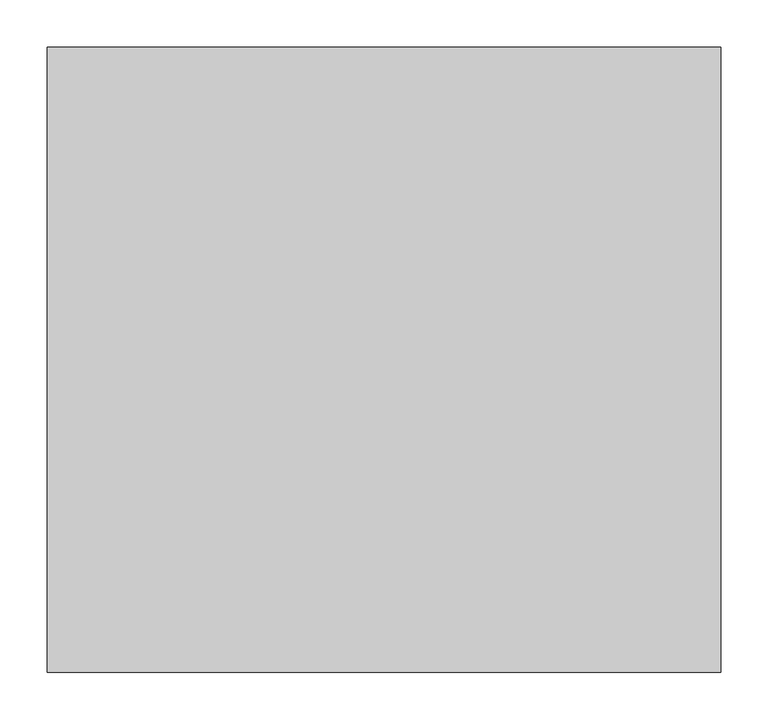
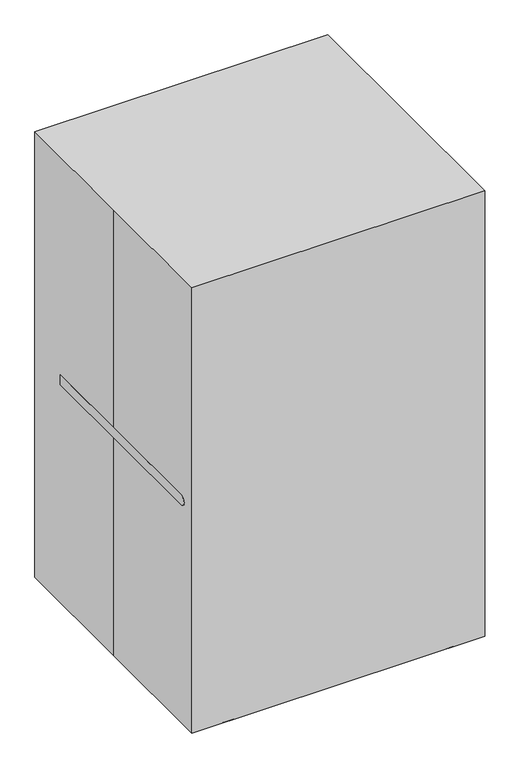
"""IFC4 building model written with IfcOpenShell, lengths in millimetres: proxy geometry, F0270 - Chair, Rocking, High Back : F0270 - Chair, Rocking, High Back."""

import ifcopenshell
import ifcopenshell.guid

model = None  # the IFC model being written
_history = None  # IfcOwnerHistory: only IFC2X3 demands one
_inside = {}  # id of a spatial element -> (the spatial element, [elements in it])
_under = {}  # id of a project, library or spatial element -> (it, [spatial elements below it])
_declared = {}  # id of a project -> (the project, [libraries it declares])
_typed = {}  # id of a type object -> (the type object, [elements of that type])
_made_of = {}  # id of a material, layer set ... -> (it, [elements and type objects made of it])


def new_model(schema):
    """Start an empty IFC model of exactly this schema.

    Asked for "IFC4X3", IfcOpenShell would pick the latest addendum, in which some entities
    have other attributes; the version numbers below select the first issue.
    IFC2X3 requires an IfcOwnerHistory on every rooted entity: one is made here for all.
    """
    global model, _history
    if schema == "IFC4X3":
        model = ifcopenshell.file(schema_version=(4, 3, 0, 0))
    else:
        model = ifcopenshell.file(schema=schema)
    _inside.clear()
    _under.clear()
    _declared.clear()
    _typed.clear()
    _made_of.clear()
    _history = None
    if model.schema == "IFC2X3":
        org = make("IfcOrganization", Name="unknown")
        user = make(
            "IfcPersonAndOrganization",
            ThePerson=make("IfcPerson", FamilyName="unknown"),
            TheOrganization=org,
        )
        app = make(
            "IfcApplication",
            ApplicationDeveloper=org,
            Version="unknown",
            ApplicationFullName="unknown",
            ApplicationIdentifier="unknown",
        )
        _history = make(
            "IfcOwnerHistory",
            OwningUser=user,
            OwningApplication=app,
            ChangeAction="ADDED",
            CreationDate=0,
        )
    return model


def make(cls, **values):
    """One entity of the class cls with the attributes given. An attribute that is None is left unset."""
    return model.create_entity(
        cls, **{name: value for name, value in values.items() if value is not None}
    )


def rooted(cls, **values):
    """An entity with a GlobalId (a new one), such as an element, a storey or a relation."""
    return make(cls, GlobalId=ifcopenshell.guid.new(), OwnerHistory=_history, **values)


def si_unit(unit_type, name, prefix=None):
    """IfcSIUnit, for example si_unit("LENGTHUNIT", "METRE", prefix="MILLI")."""
    return make("IfcSIUnit", UnitType=unit_type, Prefix=prefix, Name=name)


def assignment(units):
    """IfcUnitAssignment: the units of a project."""
    return None if units is None else make("IfcUnitAssignment", Units=units)


def point(xyz):
    """IfcCartesianPoint."""
    return None if xyz is None else make("IfcCartesianPoint", Coordinates=xyz)


def direction(xyz):
    """IfcDirection."""
    return None if xyz is None else make("IfcDirection", DirectionRatios=xyz)


def frame(location, z_axis=None, x_axis=None):
    """IfcAxis2Placement3D, a coordinate frame: its origin and axes. An axis left out is left unset."""
    return make(
        "IfcAxis2Placement3D",
        Location=point(location),
        Axis=direction(z_axis),
        RefDirection=direction(x_axis),
    )


def frame_2d(location, x_axis=None):
    """IfcAxis2Placement2D, a coordinate frame in the plane: its origin and x axis."""
    return make(
        "IfcAxis2Placement2D", Location=point(location), RefDirection=direction(x_axis)
    )


def origin():
    """The frame at (0, 0, 0) with its axes left unset."""
    return frame((0.0, 0.0, 0.0))


def origin_with_axes():
    """The frame at (0, 0, 0) with the z axis (0, 0, 1) and the x axis (1, 0, 0) written out."""
    return frame((0.0, 0.0, 0.0), z_axis=(0.0, 0.0, 1.0), x_axis=(1.0, 0.0, 0.0))


def place(relative_to, where):
    """IfcLocalPlacement: puts the frame where relative to a parent placement (None: the world)."""
    return make(
        "IfcLocalPlacement", PlacementRelTo=relative_to, RelativePlacement=where
    )


def context(
    kind, dimensions, precision=None, world=None, true_north=None, identifier=None
):
    """IfcGeometricRepresentationContext, for example the 3D "Model" context."""
    return make(
        "IfcGeometricRepresentationContext",
        ContextIdentifier=identifier,
        ContextType=kind,
        CoordinateSpaceDimension=dimensions,
        Precision=precision,
        WorldCoordinateSystem=world,
        TrueNorth=true_north,
    )


def project(units=None, contexts=None):
    """IfcProject with its units and contexts."""
    return rooted(
        "IfcProject",
        Name="project",
        RepresentationContexts=contexts,
        UnitsInContext=assignment(units),
    )


def spatial(cls, under=None, at=None, **own):
    """A site, building, storey or space (cls), placed at a placement, below another one or the project."""
    s = rooted(cls, ObjectPlacement=at, **own)
    if under is not None:
        _under.setdefault(under.id(), (under, []))[1].append(s)
    return s


def polyline(points):
    """IfcPolyline through the points."""
    return make("IfcPolyline", Points=[point(p) for p in points])


def circle_curve(where, radius):
    """IfcCircle in the frame where."""
    return make("IfcCircle", Position=where, Radius=radius)


def trimmed(basis, trim1, trim2, sense, master):
    """IfcTrimmedCurve: the piece of a basis curve between two trims."""
    return make(
        "IfcTrimmedCurve",
        BasisCurve=basis,
        Trim1=trim1,
        Trim2=trim2,
        SenseAgreement=sense,
        MasterRepresentation=master,
    )


def segment(curve, same_sense, transition):
    """IfcCompositeCurveSegment."""
    return make(
        "IfcCompositeCurveSegment",
        Transition=transition,
        SameSense=same_sense,
        ParentCurve=curve,
    )


def composite_curve(segments, self_intersect=None):
    """IfcCompositeCurve: segments joined end to end."""
    return make("IfcCompositeCurve", Segments=segments, SelfIntersect=self_intersect)


def outline(outer, holes=None, kind="AREA"):
    """IfcArbitraryClosedProfileDef: a profile drawn as a closed curve; with holes, ...WithVoids."""
    if holes is None:
        return make("IfcArbitraryClosedProfileDef", ProfileType=kind, OuterCurve=outer)
    return make(
        "IfcArbitraryProfileDefWithVoids",
        ProfileType=kind,
        OuterCurve=outer,
        InnerCurves=holes,
    )


def extrude(swept, where, along, depth):
    """IfcExtrudedAreaSolid: the profile swept, set in the frame where, extruded along a direction by depth."""
    return make(
        "IfcExtrudedAreaSolid",
        SweptArea=swept,
        Position=where,
        ExtrudedDirection=direction(along),
        Depth=depth,
    )


def shape(context_of_items, identifier, shape_type, items):
    """IfcShapeRepresentation: the items that make up one representation, for example the "Body"."""
    return make(
        "IfcShapeRepresentation",
        ContextOfItems=context_of_items,
        RepresentationIdentifier=identifier,
        RepresentationType=shape_type,
        Items=items,
    )


def source(mapping_origin, context_of_items, identifier, shape_type, items):
    """IfcRepresentationMap: a shape defined once, which mapped items show again and again."""
    return make(
        "IfcRepresentationMap",
        MappingOrigin=mapping_origin,
        MappedRepresentation=shape(context_of_items, identifier, shape_type, items),
    )


def transform(
    local_origin,
    x_axis=None,
    y_axis=None,
    z_axis=None,
    scale=None,
    scale2=None,
    scale3=None,
    uniform=True,
):
    """IfcCartesianTransformationOperator3D, or its non-uniform kind. x_axis, y_axis, z_axis: its Axis1, 2, 3."""
    if uniform:
        return make(
            "IfcCartesianTransformationOperator3D",
            Axis1=direction(x_axis),
            Axis2=direction(y_axis),
            LocalOrigin=point(local_origin),
            Scale=scale,
            Axis3=direction(z_axis),
        )
    return make(
        "IfcCartesianTransformationOperator3DnonUniform",
        Axis1=direction(x_axis),
        Axis2=direction(y_axis),
        LocalOrigin=point(local_origin),
        Scale=scale,
        Axis3=direction(z_axis),
        Scale2=scale2,
        Scale3=scale3,
    )


def mapped(mapping_source, mapping_target):
    """IfcMappedItem: shows the shape of a source again, moved by a transform."""
    return make(
        "IfcMappedItem", MappingSource=mapping_source, MappingTarget=mapping_target
    )


def made_of(thing, what):
    """Note that an element or type object is made of a material, layer set ...; save() writes the relation."""
    if what is not None:
        _made_of.setdefault(what.id(), (what, []))[1].append(thing)
    return thing


def element(
    cls,
    number,
    at=None,
    inside=None,
    cuts=None,
    type_object=None,
    material=None,
    context=None,
    identifier="Body",
    shape_type=None,
    held_by="IfcProductDefinitionShape",
    body=None,
    shapes=None,
    **own,
):
    """One element of the class cls, such as IfcWall. Its Tag is "e" and its number.

    at: its placement. inside: the storey or other place that contains it. cuts: it is an
    opening in that element (IfcRelVoidsElement). A single representation is given by context,
    identifier, shape_type and body (its items); several are given by shapes. held_by: the class
    of the entity that holds the representations. save() writes the other relations.
    """
    e = rooted(cls, Tag="e%d" % number, ObjectPlacement=at, **own)
    if body is not None:
        shapes = [shape(context, identifier, shape_type, body)]
    if shapes is not None:
        e.Representation = make(held_by, Representations=shapes)
    if inside is not None:
        _inside.setdefault(inside.id(), (inside, []))[1].append(e)
    if cuts is not None:
        rooted(
            "IfcRelVoidsElement", RelatingBuildingElement=cuts, RelatedOpeningElement=e
        )
    if type_object is not None:
        _typed.setdefault(type_object.id(), (type_object, []))[1].append(e)
    return made_of(e, material)


def aggregate(whole, parts):
    """IfcRelAggregates: a whole, such as a stair, and the parts it consists of."""
    return rooted("IfcRelAggregates", RelatingObject=whole, RelatedObjects=parts)


def save(model, path):
    """Write the relations noted so far, then the file.

    IfcRelAggregates (storeys below a building ...), IfcRelContainedInSpatialStructure (elements
    in a storey), IfcRelDefinesByType, IfcRelAssociatesMaterial and IfcRelDeclares: one each for
    every whole, place, type object, material and project.
    """
    for whole, parts in _under.values():
        aggregate(whole, parts)
    for where, things in _inside.values():
        rooted(
            "IfcRelContainedInSpatialStructure",
            RelatedElements=things,
            RelatingStructure=where,
        )
    for kind, things in _typed.values():
        rooted("IfcRelDefinesByType", RelatedObjects=things, RelatingType=kind)
    for what, things in _made_of.values():
        rooted("IfcRelAssociatesMaterial", RelatedObjects=things, RelatingMaterial=what)
    for by, libraries in _declared.values():
        rooted("IfcRelDeclares", RelatingContext=by, RelatedDefinitions=libraries)
    model.write(path)


def specialty_equipment_62103501(model_context):
    return source(origin(), model_context, "Body", "SweptSolid", [
        extrude(outline(polyline([(51.1608426, 279.3620973), (260.35, 279.3620973), (260.35, 228.5620973), (25.4, 228.5620973), (25.4, 253.9620973), (51.1608426, 253.9620973), (51.1608426, 279.3620973)])), frame((0.0, -195.0719564, 0.0), z_axis=(0.0, 1.0, 0.0), x_axis=(0.0, 0.0, 1.0)), (0.0, 0.0, 1.0), 335.8487477),
        extrude(outline(polyline([(51.1608426, -279.3620973), (51.1608426, -253.9620973), (25.4, -253.9620973), (25.4, -228.5620973), (260.35, -228.5620973), (260.35, -279.3620973), (51.1608426, -279.3620973)])), frame((0.0, -195.0719564, 0.0), z_axis=(0.0, 1.0, 0.0), x_axis=(0.0, 0.0, 1.0)), (0.0, 0.0, 1.0), 335.8487477),
        extrude(outline(polyline([(0.0, -17.4625001), (0.0, 0.0), (457.1241946, 0.0), (457.1241946, -17.4625001), (0.0, -17.4625001)])), frame((228.5620973, 69.8141966, 105.1526289), z_axis=(0.0, 0.6050832675335499, 0.7961621941231086), x_axis=(-1.0, 0.0, 0.0)), (0.0, 0.0, 1.0), 93.8711689),
        extrude(outline(polyline([(0.0, -17.4625), (0.0, 0.0), (457.1241946, 0.0), (457.1241946, -17.4625), (0.0, -17.4625)])), frame((228.5620973, -129.0090984, 91.0377454), z_axis=(0.0, -0.6050832675335499, 0.7961621941231086), x_axis=(-1.0, 0.0, 0.0)), (0.0, 0.0, 1.0), 98.3283222),
        extrude(outline(composite_curve([segment(polyline([(-254.0, 0.0), (-330.2, 0.0)]), True, "CONTINUOUS"), segment(trimmed(circle_curve(frame_2d((-232.280998, -68.1253356)), 119.2861782), [point((-330.2, 0.0))], [point((-223.0097057, 50.8))], False, "CARTESIAN"), True, "CONTINUOUS"), segment(polyline([(-223.0097057, 50.8), (178.5528819, 50.8)]), True, "CONTINUOUS"), segment(trimmed(circle_curve(frame_2d((185.0313755, -61.8388426)), 112.8249961), [point((178.5528819, 50.8))], [point((279.4, 0.0))], False, "CARTESIAN"), True, "CONTINUOUS"), segment(polyline([(279.4, 0.0), (203.2, 0.0)]), True, "CONTINUOUS"), segment(trimmed(circle_curve(frame_2d((-25.4, -1804.0054931)), 1818.4316812), [point((203.2, 0.0))], [point((-254.0, 0.0))], True, "CARTESIAN"), True, "CONTINUOUS")], self_intersect=False)), frame((253.9620973, 0.0, 0.0), z_axis=(1.0, 0.0, 0.0), x_axis=(0.0, 1.0, 0.0)), (0.0, 0.0, 1.0), 25.4),
        extrude(outline(composite_curve([segment(polyline([(-254.0, 0.0), (-330.2, 0.0)]), True, "CONTINUOUS"), segment(trimmed(circle_curve(frame_2d((-232.280998, -68.1253356)), 119.2861782), [point((-330.2, 0.0))], [point((-223.0097057, 50.8))], False, "CARTESIAN"), True, "CONTINUOUS"), segment(polyline([(-223.0097057, 50.8), (178.5528819, 50.8)]), True, "CONTINUOUS"), segment(trimmed(circle_curve(frame_2d((185.0313755, -61.8388426)), 112.8249961), [point((178.5528819, 50.8))], [point((279.4, 0.0))], False, "CARTESIAN"), True, "CONTINUOUS"), segment(polyline([(279.4, 0.0), (203.2, 0.0)]), True, "CONTINUOUS"), segment(trimmed(circle_curve(frame_2d((-25.4, -1804.0054931)), 1818.4316812), [point((203.2, 0.0))], [point((-254.0, 0.0))], True, "CARTESIAN"), True, "CONTINUOUS")], self_intersect=False)), frame((-279.3620973, 0.0, 0.0), z_axis=(1.0, 0.0, 0.0), x_axis=(0.0, 1.0, 0.0)), (0.0, 0.0, 1.0), 25.4),
        extrude(outline(composite_curve([segment(polyline([(224.0631045, 359.2938458), (224.0631045, 584.2), (179.8829848, 584.2), (248.0023304, 1058.8090608)]), True, "CONTINUOUS"), segment(trimmed(circle_curve(frame_2d((298.2870362, 1051.591834)), 50.8), [point((248.0023304, 1058.8090608))], [point((298.2870362, 1102.391834))], False, "CARTESIAN"), True, "CONTINUOUS"), segment(polyline([(298.2870362, 1102.391834), (305.0576471, 1102.391834), (330.2, 1098.7832206), (224.0631045, 359.2938458)]), True, "CONTINUOUS")], self_intersect=False)), frame((279.3620973, 0.0, 0.0), z_axis=(1.0, 0.0, 0.0), x_axis=(0.0, 1.0, 0.0)), (0.0, 0.0, 1.0), 25.4),
        extrude(outline(composite_curve([segment(polyline([(208.8094279, 431.8), (196.85, 431.8), (158.75, 431.8)]), True, "CONTINUOUS"), segment(trimmed(circle_curve(frame_2d((158.75, 455.3424503)), 23.5424503), [point((158.75, 431.8))], [point((135.2075497, 455.3424503))], False, "CARTESIAN"), True, "CONTINUOUS"), segment(polyline([(135.2075497, 455.3424503), (226.021975, 1088.0753214)]), True, "CONTINUOUS"), segment(trimmed(circle_curve(frame_2d((263.7355043, 1082.6624012)), 38.1), [point((226.021975, 1088.0753214))], [point((301.4490337, 1077.2494811))], False, "CARTESIAN"), True, "CONTINUOUS"), segment(polyline([(301.4490337, 1077.2494811), (208.8094279, 431.8)]), True, "CONTINUOUS")], self_intersect=False)), frame((-279.3620973, 0.0, 0.0), z_axis=(1.0, 0.0, 0.0), x_axis=(0.0, 1.0, 0.0)), (0.0, 0.0, 1.0), 558.7241946),
        extrude(outline(composite_curve([segment(trimmed(circle_curve(frame_2d((-284.4670631, 571.5)), 12.7), [point((-284.4670631, 558.8))], [point((-284.4670631, 584.2))], False, "CARTESIAN"), True, "CONTINUOUS"), segment(polyline([(-284.4670631, 584.2), (223.5329369, 584.2), (223.5329369, 558.8), (-284.4670631, 558.8)]), True, "CONTINUOUS")], self_intersect=False)), frame((279.3620973, 0.0, 0.0), z_axis=(1.0, 0.0, 0.0), x_axis=(0.0, 1.0, 0.0)), (0.0, 0.0, 1.0), 76.2),
        extrude(outline(composite_curve([segment(trimmed(circle_curve(frame_2d((317.4620973, 210.8329369)), 12.7), [point((330.1620973, 210.8329369))], [point((304.7620973, 210.8329369))], False, "CARTESIAN"), True, "CONTINUOUS"), segment(trimmed(circle_curve(frame_2d((317.4620973, 210.8329369)), 12.7), [point((304.7620973, 210.8329369))], [point((330.1620973, 210.8329369))], False, "CARTESIAN"), True, "CONTINUOUS")], self_intersect=False)), frame((0.0, 0.0, 355.6), z_axis=(0.0, 0.0, 1.0), x_axis=(1.0, 0.0, 0.0)), (0.0, 0.0, 1.0), 203.2),
        extrude(outline(composite_curve([segment(trimmed(circle_curve(frame_2d((317.4620973, 58.4329369)), 12.7), [point((330.1620973, 58.4329369))], [point((304.7620973, 58.4329369))], False, "CARTESIAN"), True, "CONTINUOUS"), segment(trimmed(circle_curve(frame_2d((317.4620973, 58.4329369)), 12.7), [point((304.7620973, 58.4329369))], [point((330.1620973, 58.4329369))], False, "CARTESIAN"), True, "CONTINUOUS")], self_intersect=False)), frame((0.0, 0.0, 355.6), z_axis=(0.0, 0.0, 1.0), x_axis=(1.0, 0.0, 0.0)), (0.0, 0.0, 1.0), 203.2),
        extrude(outline(composite_curve([segment(trimmed(circle_curve(frame_2d((317.4620973, -93.9670631)), 12.7), [point((330.1620973, -93.9670631))], [point((304.7620973, -93.9670631))], False, "CARTESIAN"), True, "CONTINUOUS"), segment(trimmed(circle_curve(frame_2d((317.4620973, -93.9670631)), 12.7), [point((304.7620973, -93.9670631))], [point((330.1620973, -93.9670631))], False, "CARTESIAN"), True, "CONTINUOUS")], self_intersect=False)), frame((0.0, 0.0, 355.6), z_axis=(0.0, 0.0, 1.0), x_axis=(1.0, 0.0, 0.0)), (0.0, 0.0, 1.0), 203.2),
        extrude(outline(composite_curve([segment(trimmed(circle_curve(frame_2d((317.4620973, -246.3670631)), 12.7), [point((330.1620973, -246.3670631))], [point((304.7620973, -246.3670631))], False, "CARTESIAN"), True, "CONTINUOUS"), segment(trimmed(circle_curve(frame_2d((317.4620973, -246.3670631)), 12.7), [point((304.7620973, -246.3670631))], [point((330.1620973, -246.3670631))], False, "CARTESIAN"), True, "CONTINUOUS")], self_intersect=False)), frame((0.0, 0.0, 355.6), z_axis=(0.0, 0.0, 1.0), x_axis=(1.0, 0.0, 0.0)), (0.0, 0.0, 1.0), 203.2),
        extrude(outline(composite_curve([segment(polyline([(130.1715881, 25.4), (-22.2284119, 25.4), (-174.6284119, 25.4)]), True, "CONTINUOUS"), segment(trimmed(circle_curve(frame_2d((-128.8108028, 171.45)), 153.068141), [point((-174.6284119, 25.4))], [point((-174.6284119, 317.5))], False, "CARTESIAN"), True, "CONTINUOUS"), segment(polyline([(-174.6284119, 317.5), (-22.2284119, 317.5), (130.1715881, 317.5)]), True, "CONTINUOUS"), segment(trimmed(circle_curve(frame_2d((84.353979, 171.45)), 153.068141), [point((130.1715881, 317.5))], [point((130.1715881, 25.4))], False, "CARTESIAN"), True, "CONTINUOUS")], self_intersect=False)), frame((279.3620973, 0.0, 0.0), z_axis=(1.0, 0.0, 0.0), x_axis=(0.0, 1.0, 0.0)), (0.0, 0.0, 1.0), 25.4),
        extrude(outline(composite_curve([segment(polyline([(224.0631045, 359.2938458), (224.0631045, 584.2), (179.8829848, 584.2), (248.0023304, 1058.8090608)]), True, "CONTINUOUS"), segment(trimmed(circle_curve(frame_2d((298.2870362, 1051.591834)), 50.8), [point((248.0023304, 1058.8090608))], [point((298.2870362, 1102.391834))], False, "CARTESIAN"), True, "CONTINUOUS"), segment(polyline([(298.2870362, 1102.391834), (305.0576471, 1102.391834), (330.2, 1098.7832206), (224.0631045, 359.2938458)]), True, "CONTINUOUS")], self_intersect=False)), frame((-304.7620973, 0.0, 0.0), z_axis=(1.0, 0.0, 0.0), x_axis=(0.0, 1.0, 0.0)), (0.0, 0.0, 1.0), 25.4),
        extrude(outline(polyline([(330.2, 1098.7832206), (223.5329369, 355.6), (197.8726495, 355.6), (305.0576471, 1102.391834), (330.2, 1098.7832206)])), frame((-279.3620973, 0.0, 0.0), z_axis=(1.0, 0.0, 0.0), x_axis=(0.0, 1.0, 0.0)), (0.0, 0.0, 1.0), 558.7241946),
        extrude(outline(composite_curve([segment(polyline([(-12.7, 431.8), (196.85, 431.8), (196.85, 355.6), (-12.7, 355.6), (-273.05, 355.6)]), True, "CONTINUOUS"), segment(trimmed(circle_curve(frame_2d((-273.05, 393.7)), 38.1), [point((-273.05, 355.6))], [point((-273.05, 431.8))], False, "CARTESIAN"), True, "CONTINUOUS"), segment(polyline([(-273.05, 431.8), (-12.7, 431.8)]), True, "CONTINUOUS")], self_intersect=False)), frame((-279.3620973, 0.0, 0.0), z_axis=(1.0, 0.0, 0.0), x_axis=(0.0, 1.0, 0.0)), (0.0, 0.0, 1.0), 558.7241946),
        extrude(outline(composite_curve([segment(trimmed(circle_curve(frame_2d((-284.4670631, 571.5)), 12.7), [point((-284.4670631, 558.8))], [point((-284.4670631, 584.2))], False, "CARTESIAN"), True, "CONTINUOUS"), segment(polyline([(-284.4670631, 584.2), (223.5329369, 584.2), (223.5329369, 558.8), (-284.4670631, 558.8)]), True, "CONTINUOUS")], self_intersect=False)), frame((-355.5620973, 0.0, 0.0), z_axis=(1.0, 0.0, 0.0), x_axis=(0.0, 1.0, 0.0)), (0.0, 0.0, 1.0), 76.2),
        extrude(outline(composite_curve([segment(trimmed(circle_curve(frame_2d((-317.4620973, 210.8329369)), 12.7), [point((-330.1620973, 210.8329369))], [point((-304.7620973, 210.8329369))], False, "CARTESIAN"), True, "CONTINUOUS"), segment(trimmed(circle_curve(frame_2d((-317.4620973, 210.8329369)), 12.7), [point((-304.7620973, 210.8329369))], [point((-330.1620973, 210.8329369))], False, "CARTESIAN"), True, "CONTINUOUS")], self_intersect=False)), frame((0.0, 0.0, 355.6), z_axis=(0.0, 0.0, 1.0), x_axis=(1.0, 0.0, 0.0)), (0.0, 0.0, 1.0), 203.2),
        extrude(outline(composite_curve([segment(trimmed(circle_curve(frame_2d((-317.4620973, 58.4329369)), 12.7), [point((-330.1620973, 58.4329369))], [point((-304.7620973, 58.4329369))], False, "CARTESIAN"), True, "CONTINUOUS"), segment(trimmed(circle_curve(frame_2d((-317.4620973, 58.4329369)), 12.7), [point((-304.7620973, 58.4329369))], [point((-330.1620973, 58.4329369))], False, "CARTESIAN"), True, "CONTINUOUS")], self_intersect=False)), frame((0.0, 0.0, 355.6), z_axis=(0.0, 0.0, 1.0), x_axis=(1.0, 0.0, 0.0)), (0.0, 0.0, 1.0), 203.2),
        extrude(outline(composite_curve([segment(trimmed(circle_curve(frame_2d((-317.4620973, -93.9670631)), 12.7), [point((-330.1620973, -93.9670631))], [point((-304.7620973, -93.9670631))], False, "CARTESIAN"), True, "CONTINUOUS"), segment(trimmed(circle_curve(frame_2d((-317.4620973, -93.9670631)), 12.7), [point((-304.7620973, -93.9670631))], [point((-330.1620973, -93.9670631))], False, "CARTESIAN"), True, "CONTINUOUS")], self_intersect=False)), frame((0.0, 0.0, 355.6), z_axis=(0.0, 0.0, 1.0), x_axis=(1.0, 0.0, 0.0)), (0.0, 0.0, 1.0), 203.2),
        extrude(outline(composite_curve([segment(trimmed(circle_curve(frame_2d((-317.4620973, -246.3670631)), 12.7), [point((-330.1620973, -246.3670631))], [point((-304.7620973, -246.3670631))], False, "CARTESIAN"), True, "CONTINUOUS"), segment(trimmed(circle_curve(frame_2d((-317.4620973, -246.3670631)), 12.7), [point((-304.7620973, -246.3670631))], [point((-330.1620973, -246.3670631))], False, "CARTESIAN"), True, "CONTINUOUS")], self_intersect=False)), frame((0.0, 0.0, 355.6), z_axis=(0.0, 0.0, 1.0), x_axis=(1.0, 0.0, 0.0)), (0.0, 0.0, 1.0), 203.2),
        extrude(outline(polyline([(355.6, 254.0), (355.6, -304.8), (-330.1620973, -304.8), (-330.1620973, 254.0), (355.6, 254.0)])), frame((0.0, 0.0, 317.5), z_axis=(0.0, 0.0, 1.0), x_axis=(1.0, 0.0, 0.0)), (0.0, 0.0, 1.0), 38.1),
        extrude(outline(composite_curve([segment(polyline([(130.1715881, 25.4), (-22.2284119, 25.4), (-174.6284119, 25.4)]), True, "CONTINUOUS"), segment(trimmed(circle_curve(frame_2d((-128.8108028, 171.45)), 153.068141), [point((-174.6284119, 25.4))], [point((-174.6284119, 317.5))], False, "CARTESIAN"), True, "CONTINUOUS"), segment(polyline([(-174.6284119, 317.5), (-22.2284119, 317.5), (130.1715881, 317.5)]), True, "CONTINUOUS"), segment(trimmed(circle_curve(frame_2d((84.353979, 171.45)), 153.068141), [point((130.1715881, 317.5))], [point((130.1715881, 25.4))], False, "CARTESIAN"), True, "CONTINUOUS")], self_intersect=False)), frame((-304.7620973, 0.0, 0.0), z_axis=(1.0, 0.0, 0.0), x_axis=(0.0, 1.0, 0.0)), (0.0, 0.0, 1.0), 25.4),
        extrude(outline(polyline([(-355.6, 330.2), (355.6, 330.2), (355.6, -330.2), (-355.6, -330.2), (-355.6, 0.0), (-355.6, 330.2)])), origin_with_axes(), (0.0, 0.0, 1.0), 1143.0),
    ])


if __name__ == "__main__":
    model = new_model("IFC4")
    model_context = context("Model", 3, world=origin())
    ifc_project = project(units=[si_unit("LENGTHUNIT", "METRE", prefix="MILLI")], contexts=[model_context])
    site = spatial("IfcSite", under=ifc_project)
    building = spatial("IfcBuilding", under=site)
    placement = place(None, origin())
    specialty_equipment_shape = specialty_equipment_62103501(model_context)
    element("IfcBuildingElementProxy", 1, Name="F0270 - Chair, Rocking, High Back : F0270 - Chair, Rocking, High Back", ObjectType="F0270 - Chair, Rocking, High Back : F0270 - Chair, Rocking, High Back", at=placement, inside=building, context=model_context, shape_type="MappedRepresentation", body=[
        mapped(specialty_equipment_shape, transform((0.0, 0.0, 0.0), x_axis=(1.0, 0.0, 0.0), y_axis=(0.0, 1.0, 0.0), z_axis=(0.0, 0.0, 1.0))),
    ])
    save(model, "model.ifc")

# Revit data of these elements
# Project information
#   Room Abbreviation = "NYUN2"
#   Room Description = "Bedroom, NICU, Multiple Birth (NYUN2)"
#   Sheets - Total = "5"
#   Project Issue Date = "Issue Date"
#   Project Status = "Project Status"
#   Client Name = "Owner"
#   Project Address = "Enter address here"
#   Project Name = "Project Name"
#   Project Number = "Project Number"
#   Publication Date = "30-Jan-15"
# Type "F0270 - Chair, Rocking, High Back : F0270 - Chair, Rocking, High Back"
#   Watts2 = "0"
#   Watts1 = "0"
#   Unit_Issue = "EA"
#   UTIL_6_Misc = "-"
#   UTIL_5_NonMedGas = "-"
#   UTIL_4_MiscGas = "-"
#   UTIL_3_MedGas = "-"
#   UTIL_2_Elec = "-"
#   UTIL_1_WaterDrain = "-"
#   Nomenclature = "Chair, Rocking, High Back"
#   NSN = "7110"
#   Location [instance default] = ""
#   JSN = "F0270"
#   Fund_Source_VA = "-"
#   Fund_Source_Navy = "-"
#   Fund_Source_Army = "-"
#   Fund_Source_AF = "-"
#   ELEC_Volts2 = "0"
#   ELEC_Volts1 = "0"
#   ELEC_Phase2 = "0"
#   ELEC_Phase1 = "0"
#   ELEC_HertzSwitch = "0"
#   ELEC_HertzDependent = "0"
#   ELEC_Hertz = "0"
#   ELEC_Amps2 = "0"
#   ELEC_Amps1 = "0"
#   DetailDescription = "High back rocking chair or glider. Designed for patient comfort and support. Available with sled base or straight leg base."
#   CAT_VA = "C"
#   CAT_Navy = "C"
#   CAT_IHS = "-"
#   CAT_Army = "C"
#   CAT_AF = "C"
#   BTUperhour = "0"
#   Weight_IP = 65
#   DIM_Width_IP = 2' - 4"
#   DIM_Height_IP = 3' - 9"
#   DIM_Depth_IP = 2' - 2"
# Element 1 (IfcBuildingElementProxy, "F0270 - Chair, Rocking, High Back : F0270 - Chair, Rocking, High Back")
#   Materials on its faces: "EquipSpace"
# Materials
#   "EquipSpace": class "Unassigned", colour RGB 221 217 195, transparency 0.5
